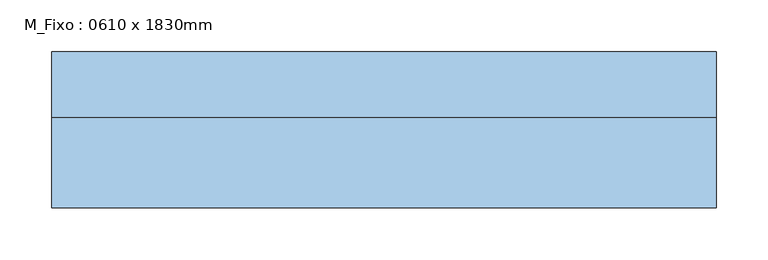
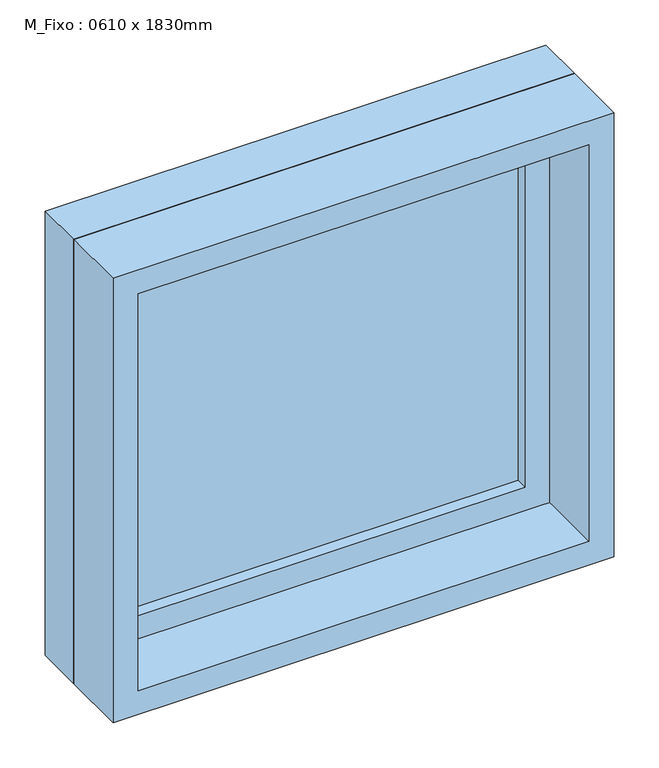
"""IFC4 building model written with IfcOpenShell, lengths in millimetres: window geometry, M_Fixo : 0610 x 1830mm."""

from ifc_helpers import new_model, si_unit, frame, origin, place, context, project, spatial, polyline, outline, extrude, source, transform, mapped, element, save


def m_fixo_0610_x_1830mm_9119c720(model_context):
    return source(origin(), model_context, "Body", "SweptSolid", [
        extrude(outline(polyline([(-257.0, 53.0), (257.0, 53.0), (257.0, 41.0), (-257.0, 41.0), (-257.0, 53.0)])), frame((0.0, 0.0, 668.0), z_axis=(0.0, 0.0, 1.0), x_axis=(1.0, 0.0, 0.0)), (0.0, 0.0, 1.0), 474.0),
        extrude(outline(polyline([(1186.0, -301.0), (624.0, -301.0), (624.0, 301.0), (1186.0, 301.0), (1186.0, -301.0)]), holes=[polyline([(1142.0, -257.0), (1142.0, 257.0), (668.0, 257.0), (668.0, -257.0), (1142.0, -257.0)])]), frame((0.0, 25.0, 0.0), z_axis=(0.0, 1.0, 0.0), x_axis=(0.0, 0.0, 1.0)), (0.0, 0.0, 1.0), 44.0),
        extrude(outline(polyline([(1205.0, -320.0), (605.0, -320.0), (605.0, 320.0), (1205.0, 320.0), (1205.0, -320.0)]), holes=[polyline([(1186.0, -301.0), (1186.0, 301.0), (624.0, 301.0), (624.0, -301.0), (1186.0, -301.0)])]), frame((0.0, 25.0, 0.0), z_axis=(0.0, 1.0, 0.0), x_axis=(0.0, 0.0, 1.0)), (0.0, 0.0, 1.0), 63.0),
        extrude(outline(polyline([(1205.0, -320.0), (605.0, -320.0), (605.0, 320.0), (1205.0, 320.0), (1205.0, -320.0)]), holes=[polyline([(1173.0, -288.0), (1173.0, 288.0), (637.0, 288.0), (637.0, -288.0), (1173.0, -288.0)])]), frame((0.0, -62.0, 0.0), z_axis=(0.0, 1.0, 0.0), x_axis=(0.0, 0.0, 1.0)), (0.0, 0.0, 1.0), 87.0),
    ])


if __name__ == "__main__":
    model = new_model("IFC4")
    model_context = context("Model", 3, world=origin())
    ifc_project = project(units=[si_unit("LENGTHUNIT", "METRE", prefix="MILLI")], contexts=[model_context])
    site = spatial("IfcSite", under=ifc_project)
    building = spatial("IfcBuilding", under=site)
    placement = place(None, origin())
    m_fixo_0610_x_1830mm_shape = m_fixo_0610_x_1830mm_9119c720(model_context)
    element("IfcWindow", 1, ObjectType="M_Fixo : 0610 x 1830mm", at=placement, inside=building, context=model_context, shape_type="MappedRepresentation", body=[
        mapped(m_fixo_0610_x_1830mm_shape, transform((0.0, 0.0, 0.0), x_axis=(1.0, 0.0, 0.0), y_axis=(0.0, 1.0, 0.0), z_axis=(0.0, 0.0, 1.0))),
    ])
    save(model, "model.ifc")

# Revit data of these elements
# Type "M_Fixo : 0610 x 1830mm"
#   Type Mark = "17"
#   Construction Type Id = "GSP4R"
#   Analytic Construction = "Vidraça única Pilkington 1/8 pol"
#   Visual Light Transmittance = 0.9
#   Thermal Resistance (R) = 0.271106 (m²·K)/W
#   Solar Heat Gain Coefficient = 0.78
#   Heat Transfer Coefficient (U) = 3.6886 W/(m²·K)
#   Height = 0.60 m
#   Altura-padrão do peitoril = 0.605 m
#   Width = 0.64 m
#   Janela aplicada = 0.019 m
#   Define Thermal Properties by = 1
#   Material da estrutura externa = Caixilho
#   Material da estrutura interna = Caixilho
#   Material do painel de vidro = Vidro
#   Caixilho = Caixilho
#   Wall Closure = (empty or 0)
# Element 1 (IfcWindow, "M_Fixo : 0610 x 1830mm")
#   Materials on its faces: "Caixilho", "Vidro"
# Materials
#   "Caixilho": class "Madeira", colour RGB 224 178 126, transparency 0, Cost = 0
#   "Vidro": class "Vidro", colour RGB 0 128 192, transparency 0.9, Description = "Vidro de sílica", Cost = 0
